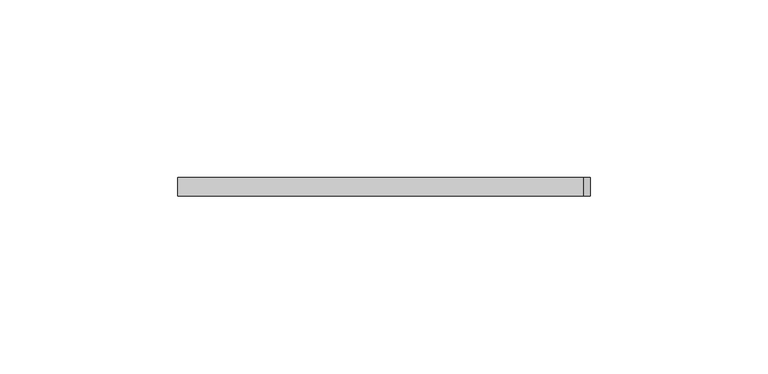
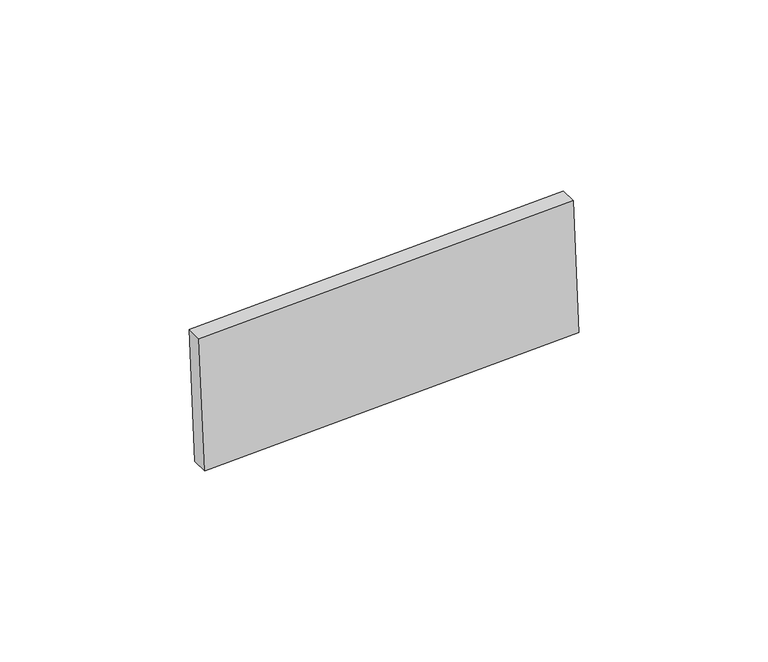
"""IFC4 building model written with IfcOpenShell, lengths in millimetres: proxy geometry, Inner panel:Inner panel:1:Inner panel:1 : Inner panel:Inner panel:300324:2:Inner panel:1:Inner panel:1 : Inner panel:Inner panel:300324:2 : Inner panel:Inner panel:1:Inner panel:1 : Inner panel:Inner panel:300324:300043:143 : Inner panel:Inner panel:1:Inner panel:1 : Inner panel:Inner panel:300324:2:Inner panel:1:Inner panel:1 : Inner panel:Inner panel:300324:2 : Inner panel:Inner panel:1:Inner panel:1 : Inner panel:Inner panel:300324:300043:308120."""

from ifc_helpers import new_model, si_unit, frame, origin, place, context, project, spatial, polyline, outline, extrude, source, transform, mapped, element, save


def generic_models_48b99092(model_context):
    return source(origin(), model_context, "Body", "SweptSolid", [
        extrude(outline(polyline([(0.0, -114.3), (0.0, 0.0), (5.2138089, 0.0), (5.2138089, -114.3), (0.0, -114.3)])), frame((558947.5116981, -578534.9848948, 3893.2872901), z_axis=(-0.04163054471216399, 0.0, 0.9991330730923527), x_axis=(0.0, -1.0, 0.0)), (0.0, 0.0, 1.0), 43.2233908),
    ])


if __name__ == "__main__":
    model = new_model("IFC4")
    model_context = context("Model", 3, world=origin())
    ifc_project = project(units=[si_unit("LENGTHUNIT", "METRE", prefix="MILLI")], contexts=[model_context])
    site = spatial("IfcSite", under=ifc_project)
    building = spatial("IfcBuilding", under=site)
    placement = place(None, origin())
    generic_models_shape = generic_models_48b99092(model_context)
    element("IfcBuildingElementProxy", 1, Name="Inner panel:Inner panel:1:Inner panel:1 : Inner panel:Inner panel:300324:2:Inner panel:1:Inner panel:1 : Inner panel:Inner panel:300324:2 : Inner panel:Inner panel:1:Inner panel:1 : Inner panel:Inner panel:300324:300043:143 : Inner panel:Inner panel:1:Inner panel:1 : Inner panel:Inner panel:300324:2:Inner panel:1:Inner panel:1 : Inner panel:Inner panel:300324:2 : Inner panel:Inner panel:1:Inner panel:1 : Inner panel:Inner panel:300324:300043:308120", ObjectType="Inner panel:Inner panel:1:Inner panel:1 : Inner panel:Inner panel:300324:2:Inner panel:1:Inner panel:1 : Inner panel:Inner panel:300324:2 : Inner panel:Inner panel:1:Inner panel:1 : Inner panel:Inner panel:300324:300043:143 : Inner panel:Inner panel:1:Inner panel:1 : Inner panel:Inner panel:300324:2:Inner panel:1:Inner panel:1 : Inner panel:Inner panel:300324:2 : Inner panel:Inner panel:1:Inner panel:1 : Inner panel:Inner panel:300324:300043:308120", at=placement, inside=building, context=model_context, shape_type="MappedRepresentation", body=[
        mapped(generic_models_shape, transform((0.0, 0.0, 0.0), x_axis=(1.0, 0.0, 0.0), y_axis=(0.0, 1.0, 0.0), z_axis=(0.0, 0.0, 1.0))),
    ])
    save(model, "model.ifc")

# Revit data of these elements
# Type "Inner panel:Inner panel:1:Inner panel:1 : Inner panel:Inner panel:300324:2:Inner panel:1:Inner panel:1 : Inner panel:Inner panel:300324:2 : Inner panel:Inner panel:1:Inner panel:1 : Inner panel:Inner panel:300324:300043:143 : Inner panel:Inner panel:1:Inner panel:1 : Inner panel:Inner panel:300324:2:Inner panel:1:Inner panel:1 : Inner panel:Inner panel:300324:2 : Inner panel:Inner panel:1:Inner panel:1 : Inner panel:Inner panel:300324:300043:308120"
#   NameOverride = "Inner panel:Inner panel:1:Inner panel:1 : Inner panel:Inner panel:300324:2:Inner panel:1:Inner panel:1 : Inner panel:Inner panel:300324:2 : Inner panel:Inner panel:1:Inner panel:1 : Inner panel:Inner panel:300324:300043:308120"
#   ObjectTypeOverride = "Inner panel:1:Inner panel:1 : Inner panel:Inner panel:300324:2 : Inner panel:Inner panel:1:Inner panel:1 : Inner panel:Inner panel:300324:300043"
#   Reference = "Inner panel"
#   Tag = "308120"
# Element 1 (IfcBuildingElementProxy, "Inner panel:Inner panel:1:Inner panel:1 : Inner panel:Inner panel:300324:2:Inner panel:1:Inner panel:1 : Inner panel:Inner panel:300324:2 : Inner panel:Inner panel:1:Inner panel:1 : Inner panel:Inner panel:300324:300043:143 : Inner panel:Inner panel:1:Inner panel:1 : Inner panel:Inner panel:300324:2:Inner panel:1:Inner panel:1 : Inner panel:Inner panel:300324:2 : Inner panel:Inner panel:1:Inner panel:1 : Inner panel:Inner panel:300324:300043:308120")
#   Materials on its faces: "SLIDING CLIP"
# Materials
#   "SLIDING CLIP": class "Generic", colour RGB 120 120 120, transparency 0, Cost = 0
